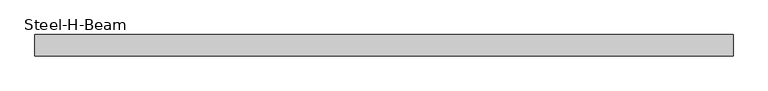
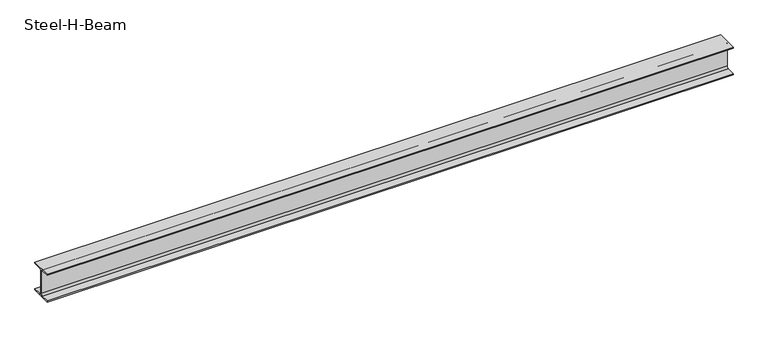
"""IFC4 building model written with IfcOpenShell, lengths in millimetres: beam geometry, Steel-H-Beam : BM121_H-244×175x7x11."""

import ifcopenshell
import ifcopenshell.guid

model = None  # the IFC model being written
_history = None  # IfcOwnerHistory: only IFC2X3 demands one
_inside = {}  # id of a spatial element -> (the spatial element, [elements in it])
_under = {}  # id of a project, library or spatial element -> (it, [spatial elements below it])
_declared = {}  # id of a project -> (the project, [libraries it declares])
_typed = {}  # id of a type object -> (the type object, [elements of that type])
_made_of = {}  # id of a material, layer set ... -> (it, [elements and type objects made of it])


def new_model(schema):
    """Start an empty IFC model of exactly this schema.

    Asked for "IFC4X3", IfcOpenShell would pick the latest addendum, in which some entities
    have other attributes; the version numbers below select the first issue.
    IFC2X3 requires an IfcOwnerHistory on every rooted entity: one is made here for all.
    """
    global model, _history
    if schema == "IFC4X3":
        model = ifcopenshell.file(schema_version=(4, 3, 0, 0))
    else:
        model = ifcopenshell.file(schema=schema)
    _inside.clear()
    _under.clear()
    _declared.clear()
    _typed.clear()
    _made_of.clear()
    _history = None
    if model.schema == "IFC2X3":
        org = make("IfcOrganization", Name="unknown")
        user = make(
            "IfcPersonAndOrganization",
            ThePerson=make("IfcPerson", FamilyName="unknown"),
            TheOrganization=org,
        )
        app = make(
            "IfcApplication",
            ApplicationDeveloper=org,
            Version="unknown",
            ApplicationFullName="unknown",
            ApplicationIdentifier="unknown",
        )
        _history = make(
            "IfcOwnerHistory",
            OwningUser=user,
            OwningApplication=app,
            ChangeAction="ADDED",
            CreationDate=0,
        )
    return model


def make(cls, **values):
    """One entity of the class cls with the attributes given. An attribute that is None is left unset."""
    return model.create_entity(
        cls, **{name: value for name, value in values.items() if value is not None}
    )


def rooted(cls, **values):
    """An entity with a GlobalId (a new one), such as an element, a storey or a relation."""
    return make(cls, GlobalId=ifcopenshell.guid.new(), OwnerHistory=_history, **values)


def si_unit(unit_type, name, prefix=None):
    """IfcSIUnit, for example si_unit("LENGTHUNIT", "METRE", prefix="MILLI")."""
    return make("IfcSIUnit", UnitType=unit_type, Prefix=prefix, Name=name)


def assignment(units):
    """IfcUnitAssignment: the units of a project."""
    return None if units is None else make("IfcUnitAssignment", Units=units)


def point(xyz):
    """IfcCartesianPoint."""
    return None if xyz is None else make("IfcCartesianPoint", Coordinates=xyz)


def direction(xyz):
    """IfcDirection."""
    return None if xyz is None else make("IfcDirection", DirectionRatios=xyz)


def frame(location, z_axis=None, x_axis=None):
    """IfcAxis2Placement3D, a coordinate frame: its origin and axes. An axis left out is left unset."""
    return make(
        "IfcAxis2Placement3D",
        Location=point(location),
        Axis=direction(z_axis),
        RefDirection=direction(x_axis),
    )


def frame_2d(location, x_axis=None):
    """IfcAxis2Placement2D, a coordinate frame in the plane: its origin and x axis."""
    return make(
        "IfcAxis2Placement2D", Location=point(location), RefDirection=direction(x_axis)
    )


def origin():
    """The frame at (0, 0, 0) with its axes left unset."""
    return frame((0.0, 0.0, 0.0))


def place(relative_to, where):
    """IfcLocalPlacement: puts the frame where relative to a parent placement (None: the world)."""
    return make(
        "IfcLocalPlacement", PlacementRelTo=relative_to, RelativePlacement=where
    )


def context(
    kind, dimensions, precision=None, world=None, true_north=None, identifier=None
):
    """IfcGeometricRepresentationContext, for example the 3D "Model" context."""
    return make(
        "IfcGeometricRepresentationContext",
        ContextIdentifier=identifier,
        ContextType=kind,
        CoordinateSpaceDimension=dimensions,
        Precision=precision,
        WorldCoordinateSystem=world,
        TrueNorth=true_north,
    )


def project(units=None, contexts=None):
    """IfcProject with its units and contexts."""
    return rooted(
        "IfcProject",
        Name="project",
        RepresentationContexts=contexts,
        UnitsInContext=assignment(units),
    )


def spatial(cls, under=None, at=None, **own):
    """A site, building, storey or space (cls), placed at a placement, below another one or the project."""
    s = rooted(cls, ObjectPlacement=at, **own)
    if under is not None:
        _under.setdefault(under.id(), (under, []))[1].append(s)
    return s


def polyline(points):
    """IfcPolyline through the points."""
    return make("IfcPolyline", Points=[point(p) for p in points])


def circle_curve(where, radius):
    """IfcCircle in the frame where."""
    return make("IfcCircle", Position=where, Radius=radius)


def trimmed(basis, trim1, trim2, sense, master):
    """IfcTrimmedCurve: the piece of a basis curve between two trims."""
    return make(
        "IfcTrimmedCurve",
        BasisCurve=basis,
        Trim1=trim1,
        Trim2=trim2,
        SenseAgreement=sense,
        MasterRepresentation=master,
    )


def segment(curve, same_sense, transition):
    """IfcCompositeCurveSegment."""
    return make(
        "IfcCompositeCurveSegment",
        Transition=transition,
        SameSense=same_sense,
        ParentCurve=curve,
    )


def composite_curve(segments, self_intersect=None):
    """IfcCompositeCurve: segments joined end to end."""
    return make("IfcCompositeCurve", Segments=segments, SelfIntersect=self_intersect)


def outline(outer, holes=None, kind="AREA"):
    """IfcArbitraryClosedProfileDef: a profile drawn as a closed curve; with holes, ...WithVoids."""
    if holes is None:
        return make("IfcArbitraryClosedProfileDef", ProfileType=kind, OuterCurve=outer)
    return make(
        "IfcArbitraryProfileDefWithVoids",
        ProfileType=kind,
        OuterCurve=outer,
        InnerCurves=holes,
    )


def extrude(swept, where, along, depth):
    """IfcExtrudedAreaSolid: the profile swept, set in the frame where, extruded along a direction by depth."""
    return make(
        "IfcExtrudedAreaSolid",
        SweptArea=swept,
        Position=where,
        ExtrudedDirection=direction(along),
        Depth=depth,
    )


def shape(context_of_items, identifier, shape_type, items):
    """IfcShapeRepresentation: the items that make up one representation, for example the "Body"."""
    return make(
        "IfcShapeRepresentation",
        ContextOfItems=context_of_items,
        RepresentationIdentifier=identifier,
        RepresentationType=shape_type,
        Items=items,
    )


def source(mapping_origin, context_of_items, identifier, shape_type, items):
    """IfcRepresentationMap: a shape defined once, which mapped items show again and again."""
    return make(
        "IfcRepresentationMap",
        MappingOrigin=mapping_origin,
        MappedRepresentation=shape(context_of_items, identifier, shape_type, items),
    )


def transform(
    local_origin,
    x_axis=None,
    y_axis=None,
    z_axis=None,
    scale=None,
    scale2=None,
    scale3=None,
    uniform=True,
):
    """IfcCartesianTransformationOperator3D, or its non-uniform kind. x_axis, y_axis, z_axis: its Axis1, 2, 3."""
    if uniform:
        return make(
            "IfcCartesianTransformationOperator3D",
            Axis1=direction(x_axis),
            Axis2=direction(y_axis),
            LocalOrigin=point(local_origin),
            Scale=scale,
            Axis3=direction(z_axis),
        )
    return make(
        "IfcCartesianTransformationOperator3DnonUniform",
        Axis1=direction(x_axis),
        Axis2=direction(y_axis),
        LocalOrigin=point(local_origin),
        Scale=scale,
        Axis3=direction(z_axis),
        Scale2=scale2,
        Scale3=scale3,
    )


def mapped(mapping_source, mapping_target):
    """IfcMappedItem: shows the shape of a source again, moved by a transform."""
    return make(
        "IfcMappedItem", MappingSource=mapping_source, MappingTarget=mapping_target
    )


def made_of(thing, what):
    """Note that an element or type object is made of a material, layer set ...; save() writes the relation."""
    if what is not None:
        _made_of.setdefault(what.id(), (what, []))[1].append(thing)
    return thing


def element(
    cls,
    number,
    at=None,
    inside=None,
    cuts=None,
    type_object=None,
    material=None,
    context=None,
    identifier="Body",
    shape_type=None,
    held_by="IfcProductDefinitionShape",
    body=None,
    shapes=None,
    **own,
):
    """One element of the class cls, such as IfcWall. Its Tag is "e" and its number.

    at: its placement. inside: the storey or other place that contains it. cuts: it is an
    opening in that element (IfcRelVoidsElement). A single representation is given by context,
    identifier, shape_type and body (its items); several are given by shapes. held_by: the class
    of the entity that holds the representations. save() writes the other relations.
    """
    e = rooted(cls, Tag="e%d" % number, ObjectPlacement=at, **own)
    if body is not None:
        shapes = [shape(context, identifier, shape_type, body)]
    if shapes is not None:
        e.Representation = make(held_by, Representations=shapes)
    if inside is not None:
        _inside.setdefault(inside.id(), (inside, []))[1].append(e)
    if cuts is not None:
        rooted(
            "IfcRelVoidsElement", RelatingBuildingElement=cuts, RelatedOpeningElement=e
        )
    if type_object is not None:
        _typed.setdefault(type_object.id(), (type_object, []))[1].append(e)
    return made_of(e, material)


def aggregate(whole, parts):
    """IfcRelAggregates: a whole, such as a stair, and the parts it consists of."""
    return rooted("IfcRelAggregates", RelatingObject=whole, RelatedObjects=parts)


def save(model, path):
    """Write the relations noted so far, then the file.

    IfcRelAggregates (storeys below a building ...), IfcRelContainedInSpatialStructure (elements
    in a storey), IfcRelDefinesByType, IfcRelAssociatesMaterial and IfcRelDeclares: one each for
    every whole, place, type object, material and project.
    """
    for whole, parts in _under.values():
        aggregate(whole, parts)
    for where, things in _inside.values():
        rooted(
            "IfcRelContainedInSpatialStructure",
            RelatedElements=things,
            RelatingStructure=where,
        )
    for kind, things in _typed.values():
        rooted("IfcRelDefinesByType", RelatedObjects=things, RelatingType=kind)
    for what, things in _made_of.values():
        rooted("IfcRelAssociatesMaterial", RelatedObjects=things, RelatingMaterial=what)
    for by, libraries in _declared.values():
        rooted("IfcRelDeclares", RelatingContext=by, RelatedDefinitions=libraries)
    model.write(path)


def steel_h_beam_2cee67ca(model_context):
    return source(origin(), model_context, "Body", "SweptSolid", [
        extrude(outline(composite_curve([segment(polyline([(87.5, -111.0), (87.5, -122.0), (-87.5, -122.0), (-87.5, -111.0), (-19.5, -111.0)]), True, "CONTINUOUS"), segment(trimmed(circle_curve(frame_2d((-19.5, -95.0)), 16.0), [point((-19.5, -111.0))], [point((-3.5, -95.0))], True, "CARTESIAN"), True, "CONTINUOUS"), segment(polyline([(-3.5, -95.0), (-3.5, 95.0)]), True, "CONTINUOUS"), segment(trimmed(circle_curve(frame_2d((-19.5, 95.0)), 16.0), [point((-3.5, 95.0))], [point((-19.5, 111.0))], True, "CARTESIAN"), True, "CONTINUOUS"), segment(polyline([(-19.5, 111.0), (-87.5, 111.0), (-87.5, 122.0), (87.5, 122.0), (87.5, 111.0), (19.5, 111.0)]), True, "CONTINUOUS"), segment(trimmed(circle_curve(frame_2d((19.5, 95.0)), 16.0), [point((19.5, 111.0))], [point((3.5, 95.0))], True, "CARTESIAN"), True, "CONTINUOUS"), segment(polyline([(3.5, 95.0), (3.5, -95.0)]), True, "CONTINUOUS"), segment(trimmed(circle_curve(frame_2d((19.5, -95.0)), 16.0), [point((3.5, -95.0))], [point((19.5, -111.0))], True, "CARTESIAN"), True, "CONTINUOUS"), segment(polyline([(19.5, -111.0), (87.5, -111.0)]), True, "CONTINUOUS")], self_intersect=False)), frame((-2886.3486745, 0.0, 0.0), z_axis=(1.0, 0.0, 0.0), x_axis=(0.0, 1.0, 0.0)), (0.0, 0.0, 1.0), 5681.8597388),
    ])


if __name__ == "__main__":
    model = new_model("IFC4")
    model_context = context("Model", 3, world=origin())
    ifc_project = project(units=[si_unit("LENGTHUNIT", "METRE", prefix="MILLI")], contexts=[model_context])
    site = spatial("IfcSite", under=ifc_project)
    building = spatial("IfcBuilding", under=site)
    placement = place(None, origin())
    steel_h_beam_shape = steel_h_beam_2cee67ca(model_context)
    element("IfcBeam", 1, ObjectType="Steel-H-Beam : BM121_H-244×175x7x11", at=placement, inside=building, context=model_context, shape_type="MappedRepresentation", body=[
        mapped(steel_h_beam_shape, transform((0.0, 0.0, 0.0), x_axis=(1.0, 0.0, 0.0), y_axis=(0.0, 1.0, 0.0), z_axis=(0.0, 0.0, 1.0))),
    ])
    save(model, "model.ifc")

# Revit data of these elements
# Type "Steel-H-Beam : BM121_H-244×175x7x11"
#   Surface Area = 1.14653 m²/m
#   Section Area = 56.2375 cm²
#   Mass per Unit Length = 44.1465 kg/m
#   Length [instance default] = 3000 mm
#   B = 175 mm
#   H = 244 mm
#   r = 16 mm
#   tw = 7 mm
#   tf = 11 mm
#   hec_material4 [instance default] = none
#   hec_material3 [instance default] = none
#   hec_material2 [instance default] = none
#   hec_material1 [instance default] = none
#   Structural Material [instance default] = Steel, 45-345
#   Assembly Code = ""
# Element 1 (IfcBeam, "Steel-H-Beam : BM121_H-244×175x7x11")
#   hec_material3 = F01AC000-00002_Building/Shelter Fire Proofing Work_Intumescent Coating Type_1 hr. rating (UL 1709))
#   hec_material2 = S01AA010-00002_Main Steel Structure Fabrication Work_Shelter/Building_Steel Painting/Coating_for Fireproofed Steel Surface, Surface Preparation & Primer Coat
#   hec_material1 = S03AA028-00001_Main Steel Structure Erection Work_Shelter/Building_Medium Steel
#   Materials on its faces: "Steel, 45-345"
# Materials
#   "Steel, 45-345": class "Metal", colour RGB 189 187 185, transparency 0, Description = "Steel 345 MPa", Cost = 0
#   "F01AC000-00002_Building/Shelter Fire Proofing Work_Intumescent Coating Type_1 hr. rating (UL 1709))": class "Metal", colour RGB 255 128 128, transparency 0, Description = "Paint finished steel", W00) Work Master Code = "F01AC000-00002", W01) Work Master_Lv1 = "Building/Shelter Fire Proofing Work", W02) Work Master_Lv2 = "Intumescent Coating Type", W03) Work Master_Spec.1 = "1 hr. rating (UL 1709)", Cost = 0
#   "S01AA010-00002_Main Steel Structure Fabrication Work_Shelter/Building_Steel Painting/Coating_for Fireproofed Steel Surface, Surface Preparation & Primer Coat": class "Metal", colour RGB 120 120 120, transparency 0, Description = "Paint finished steel", W00) Work Master Code = "SS01AA010-00002", W01) Work Master_Lv1 = "Main Steel Structure Fabrication Work", W02) Work Master_Lv2 = "Shelter/Building", W03) Work Master_Spec.1 = "Steel Painting/Coating", W04) Work Master_Spec.2 = "for Fireproofed Steel Surface, Surface Preparation & Primer Coat", Cost = 0
#   "S03AA028-00001_Main Steel Structure Erection Work_Shelter/Building_Medium Steel": class "Metal", colour RGB 120 120 120, transparency 0, Comments = "(90KG/M>Weight≥30KG/M)", Description = "Structural steel 50ksi", W00) Work Master Code = "S03AA028-0001", W01) Work Master_Lv1 = "Main Steel Structure Erection Work", W02) Work Master_Lv2 = "Shelter/Building", W03) Work Master_Spec.1 = "Medium Steel (90KG/M>Weight≥30KG/M)", Cost = 0
